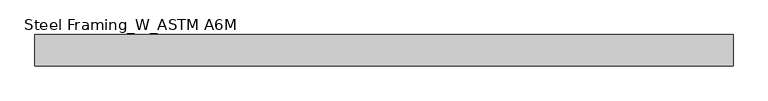
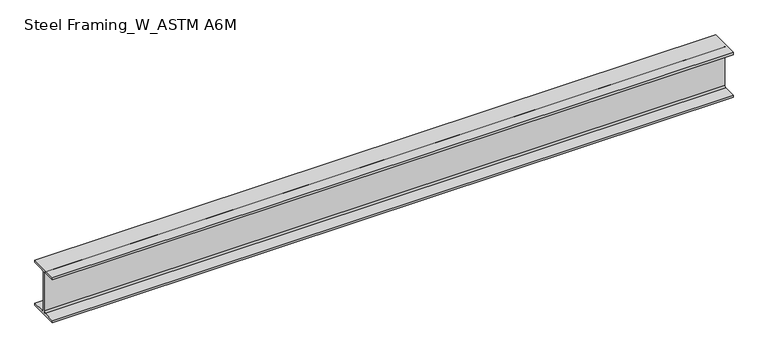
"""IFC4 building model written with IfcOpenShell, lengths in millimetres: beam geometry, Steel Framing_W_ASTM A6M : H_SB_AR_S02_W200x31.3_RB4."""

from ifc_helpers import new_model, si_unit, point, frame, frame_2d, origin, place, context, project, spatial, polyline, circle_curve, trimmed, segment, composite_curve, outline, extrude, source, transform, mapped, element, save


def steel_framing_w_astm_a6m_acb30e8c(model_context):
    return source(origin(), model_context, "Body", "SweptSolid", [
        extrude(outline(composite_curve([segment(polyline([(67.0, -94.8), (67.0, -105.0), (-67.0, -105.0), (-67.0, -94.8), (-10.775, -94.8)]), True, "CONTINUOUS"), segment(trimmed(circle_curve(frame_2d((-10.775, -87.2)), 7.6), [point((-10.775, -94.8))], [point((-3.175, -87.2))], True, "CARTESIAN"), True, "CONTINUOUS"), segment(polyline([(-3.175, -87.2), (-3.175, 87.2)]), True, "CONTINUOUS"), segment(trimmed(circle_curve(frame_2d((-10.775, 87.2)), 7.6), [point((-3.175, 87.2))], [point((-10.775, 94.8))], True, "CARTESIAN"), True, "CONTINUOUS"), segment(polyline([(-10.775, 94.8), (-67.0, 94.8), (-67.0, 105.0), (67.0, 105.0), (67.0, 94.8), (10.775, 94.8)]), True, "CONTINUOUS"), segment(trimmed(circle_curve(frame_2d((10.775, 87.2)), 7.6), [point((10.775, 94.8))], [point((3.175, 87.2))], True, "CARTESIAN"), True, "CONTINUOUS"), segment(polyline([(3.175, 87.2), (3.175, -87.2)]), True, "CONTINUOUS"), segment(trimmed(circle_curve(frame_2d((10.775, -87.2)), 7.6), [point((3.175, -87.2))], [point((10.775, -94.8))], True, "CARTESIAN"), True, "CONTINUOUS"), segment(polyline([(10.775, -94.8), (67.0, -94.8)]), True, "CONTINUOUS")], self_intersect=False)), frame((-1500.0, 0.0, 0.0), z_axis=(1.0, 0.0, 0.0), x_axis=(0.0, 1.0, 0.0)), (0.0, 0.0, 1.0), 3000.0),
    ])


if __name__ == "__main__":
    model = new_model("IFC4")
    model_context = context("Model", 3, world=origin())
    ifc_project = project(units=[si_unit("LENGTHUNIT", "METRE", prefix="MILLI")], contexts=[model_context])
    site = spatial("IfcSite", under=ifc_project)
    building = spatial("IfcBuilding", under=site)
    placement = place(None, origin())
    steel_framing_w_astm_a6m_shape = steel_framing_w_astm_a6m_acb30e8c(model_context)
    element("IfcBeam", 1, ObjectType="Steel Framing_W_ASTM A6M : H_SB_AR_S02_W200x31.3_RB4", at=placement, inside=building, context=model_context, shape_type="MappedRepresentation", body=[
        mapped(steel_framing_w_astm_a6m_shape, transform((0.0, 0.0, 0.0), x_axis=(1.0, 0.0, 0.0), y_axis=(0.0, 1.0, 0.0), z_axis=(0.0, 0.0, 1.0))),
    ])
    save(model, "model.ifc")

# Revit data of these elements
# Type "Steel Framing_W_ASTM A6M : H_SB_AR_S02_W200x31.3_RB4"
#   Type Mark = "RB4"
#   Section Name Key = "W8x21"
#   Width = 13.4 cm
#   Web Thickness = 0.635 cm
#   Web Fillet = 0.76 cm
#   Warping Constant = 40800.0 cm⁶
#   Torsional Moment of Inertia = 11.70 cm⁴
#   Section Area = 39.7 cm²
#   Plastic Modulus weak axis = 93.2 cm³
#   Plastic Modulus strong axis = 334.0 cm³
#   Perimeter = 0.93 m²/m
#   Nominal Weight = 31.30 kgf/m
#   Moment of Inertia weak axis = 407.00 cm⁴
#   Moment of Inertia strong axis = 3130.00 cm⁴
#   Height = 21.0 cm
#   Flange Thickness = 1.02 cm
#   Elastic Modulus weak axis = 60.8 cm³
#   Elastic Modulus strong axis = 298.0 cm³
#   Centroid Vertical = 10.5 cm
#   Centroid Horizontal = 6.7 cm
#   Length [instance default] = 1500 mm
#   Structural Material [instance default] = Steel, 45-345
#   Bolt Spacing = 0
#   Assembly Code = ""
# Element 1 (IfcBeam, "Steel Framing_W_ASTM A6M : H_SB_AR_S02_W200x31.3_RB4")
#   Materials on its faces: "Steel, 45-345"
# Materials
#   "Steel, 45-345": class "Metal", colour RGB 189 187 185, transparency 0, Description = "Steel 345 MPa", Cost = 0
